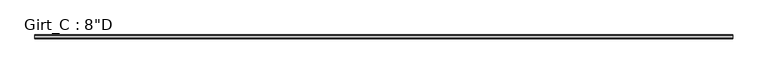
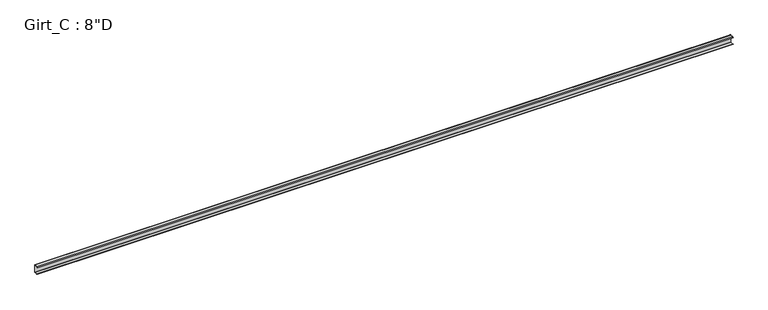
"""IFC4 building model written with IfcOpenShell, lengths in millimetres: beam geometry."""

from ifc_helpers import new_model, si_unit, point, frame, frame_2d, origin, place, context, project, spatial, polyline, circle_curve, trimmed, segment, composite_curve, outline, extrude, source, transform, mapped, element, save


def beam_c460d5f1(model_context):
    return source(origin(), model_context, "Body", "SweptSolid", [
        extrude(outline(composite_curve([segment(polyline([(-87.5109375, 101.6), (-3.3734375, 101.6)]), True, "CONTINUOUS"), segment(trimmed(circle_curve(frame_2d((-3.3734375, 96.8375)), 4.7625), [point((-3.3734375, 101.6))], [point((1.3890625, 96.8375))], False, "CARTESIAN"), True, "CONTINUOUS"), segment(polyline([(1.3890625, 96.8375), (1.3890625, -96.8375)]), True, "CONTINUOUS"), segment(trimmed(circle_curve(frame_2d((-3.3734375, -96.8375)), 4.7625), [point((1.3890625, -96.8375))], [point((-3.3734375, -101.6))], False, "CARTESIAN"), True, "CONTINUOUS"), segment(polyline([(-3.3734375, -101.6), (-87.5109375, -101.6), (-99.7792647, -86.979177), (-97.6510975, -85.1934327), (-86.2154765, -98.821875), (-3.2694106, -98.821875)]), True, "CONTINUOUS"), segment(trimmed(circle_curve(frame_2d((-3.3748024, -96.8389339)), 1.9857399), [point((-3.2694106, -98.821875))], [point((-1.3890625, -96.8389339))], True, "CARTESIAN"), True, "CONTINUOUS"), segment(polyline([(-1.3890625, -96.8389339), (-1.3890625, 96.8381931)]), True, "CONTINUOUS"), segment(trimmed(circle_curve(frame_2d((-3.3741066, 96.8381931)), 1.9850441), [point((-1.3890625, 96.8381931))], [point((-3.3005807, 98.821875))], True, "CARTESIAN"), True, "CONTINUOUS"), segment(polyline([(-3.3005807, 98.821875), (-86.2154765, 98.821875), (-97.6278742, 85.221109), (-99.7560415, 87.0068534), (-87.5109375, 101.6)]), True, "CONTINUOUS")], self_intersect=False)), frame((-8849.7913125, 0.0, 0.0), z_axis=(1.0, 0.0, 0.0), x_axis=(0.0, 1.0, 0.0)), (0.0, 0.0, 1.0), 17865.476375),
    ])


if __name__ == "__main__":
    model = new_model("IFC4")
    model_context = context("Model", 3, world=origin())
    ifc_project = project(units=[si_unit("LENGTHUNIT", "METRE", prefix="MILLI")], contexts=[model_context])
    site = spatial("IfcSite", under=ifc_project)
    building = spatial("IfcBuilding", under=site)
    placement = place(None, origin())
    beam_shape = beam_c460d5f1(model_context)
    element("IfcBeam", 1, ObjectType="Girt_C : 8\"D", at=placement, inside=building, context=model_context, shape_type="MappedRepresentation", body=[
        mapped(beam_shape, transform((0.0, 0.0, 0.0), x_axis=(1.0, 0.0, 0.0), y_axis=(0.0, 1.0, 0.0), z_axis=(0.0, 0.0, 1.0))),
    ])
    save(model, "model.ifc")

# Revit data of these elements
# Type "Girt_C : 8\"D"
#   half leg = 0' - 1 3/4"
#   Web_Thickness = 0' - 0 7/64"
#   Length [instance default] = 10' - 0"
#   Leg_1 = 0' - 3 1/2"
#   Height = 0' - 8"
#   Structural Material [instance default] = none
# Element 1 (IfcBeam, "Girt_C : 8\"D")
#   Structural Material = CEE' SECTION (8.0x3.5C - SEE STRUCT. DWGS)
#   Materials on its faces: "CEE' SECTION (8.0x3.5C - SEE STRUCT. DWGS)"
# Materials
#   "CEE' SECTION (8.0x3.5C - SEE STRUCT. DWGS)": class "Metal", colour RGB 137 146 153, transparency 0, Description = "Steel, mill finish", Cost = 0
